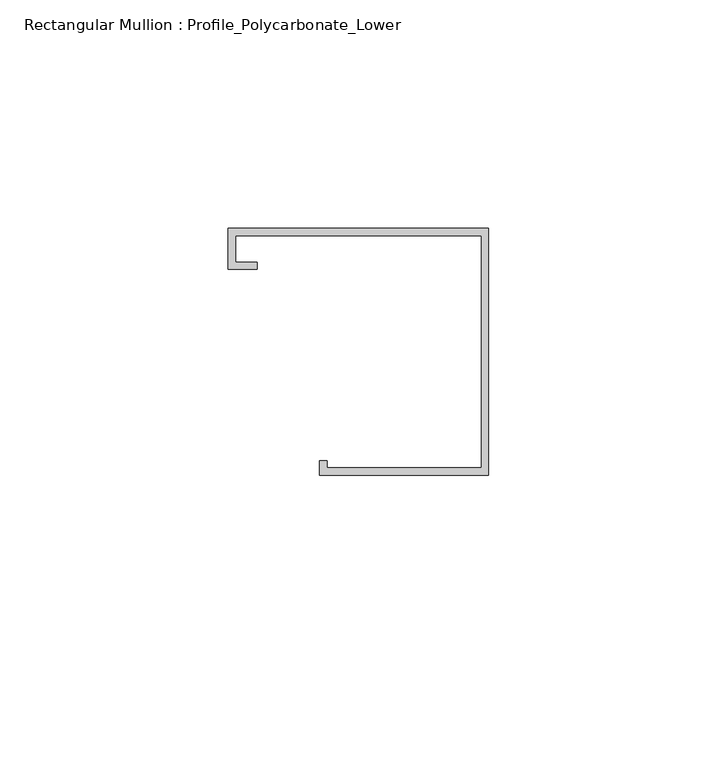
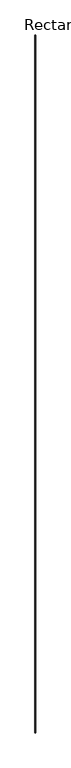
"""IFC4 building model written with IfcOpenShell, lengths in millimetres: member geometry, Rectangular Mullion : Profile_Polycarbonate_Lower."""

from ifc_helpers import new_model, si_unit, frame, origin, place, context, project, spatial, polyline, outline, extrude, source, transform, mapped, element, save


def rectangular_mullion_profile_polycarbonate_lower_36b153d9(model_context):
    return source(origin(), model_context, "Body", "SweptSolid", [
        extrude(outline(polyline([(0.0, 28.984575), (0.0, -25.015825), (-36.9824, -25.015825), (-36.9824, -21.840825), (-35.3949, -21.840825), (-35.3949, -23.428325), (-1.5875, -23.428325), (-1.5875, 27.397075), (-55.4101, 27.397075), (-55.4101, 21.580475), (-50.6476, 21.580475), (-50.6476, 19.992975), (-56.9976, 19.992975), (-56.9976, 28.984575), (0.0, 28.984575)])), frame((0.0, 0.0, -80917.7063063), z_axis=(0.0, 0.0, 1.0), x_axis=(1.0, 0.0, 0.0)), (0.0, 0.0, 1.0), 80917.7063063),
    ])


if __name__ == "__main__":
    model = new_model("IFC4")
    model_context = context("Model", 3, world=origin())
    ifc_project = project(units=[si_unit("LENGTHUNIT", "METRE", prefix="MILLI")], contexts=[model_context])
    site = spatial("IfcSite", under=ifc_project)
    building = spatial("IfcBuilding", under=site)
    placement = place(None, origin())
    rectangular_mullion_profile_polycarbonate_lower_shape = rectangular_mullion_profile_polycarbonate_lower_36b153d9(model_context)
    element("IfcMember", 1, ObjectType="Rectangular Mullion : Profile_Polycarbonate_Lower", at=placement, inside=building, context=model_context, shape_type="MappedRepresentation", body=[
        mapped(rectangular_mullion_profile_polycarbonate_lower_shape, transform((0.0, 0.0, 0.0), x_axis=(1.0, 0.0, 0.0), y_axis=(0.0, 1.0, 0.0), z_axis=(0.0, 0.0, 1.0))),
    ])
    save(model, "model.ifc")

# Revit data of these elements
# Type "Rectangular Mullion : Profile_Polycarbonate_Lower"
#   built-in parameter 1007322 = 0.177167 (stored number, unit not read)
#   built-in parameter 1007321 = 0 (stored number, unit not read)
#   built-in parameter 1007320 = 0.00520833 (stored number, unit not read)
